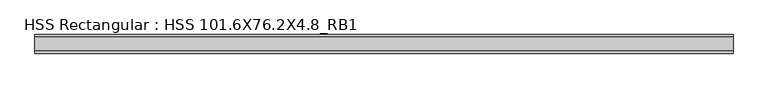
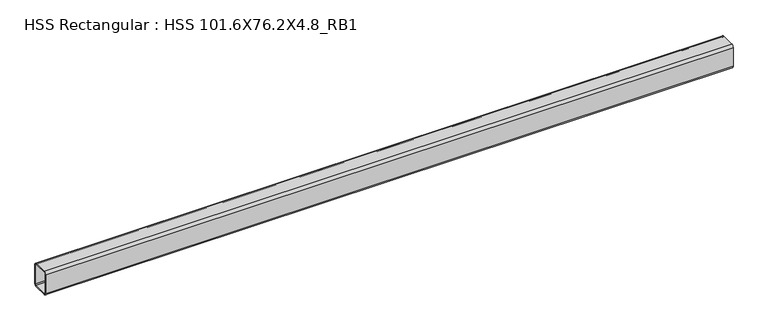
"""IFC4 building model written with IfcOpenShell, lengths in millimetres: beam geometry, HSS Rectangular : HSS 101.6X76.2X4.8_RB1."""

from ifc_helpers import new_model, si_unit, point, frame, frame_2d, origin, place, context, project, spatial, polyline, circle_curve, trimmed, segment, composite_curve, outline, extrude, source, transform, mapped, element, save


def hss_rectangular_hss_101_6x76_2x4_8_rb1_0483caaa(model_context):
    return source(origin(), model_context, "Body", "SweptSolid", [
        extrude(outline(composite_curve([segment(trimmed(circle_curve(frame_2d((-28.575, 41.275)), 9.525), [point((-38.1, 41.275))], [point((-28.575, 50.8))], False, "CARTESIAN"), True, "CONTINUOUS"), segment(polyline([(-28.575, 50.8), (28.575, 50.8)]), True, "CONTINUOUS"), segment(trimmed(circle_curve(frame_2d((28.575, 41.275)), 9.525), [point((28.575, 50.8))], [point((38.1, 41.275))], False, "CARTESIAN"), True, "CONTINUOUS"), segment(polyline([(38.1, 41.275), (38.1, -41.275)]), True, "CONTINUOUS"), segment(trimmed(circle_curve(frame_2d((28.575, -41.275)), 9.525), [point((38.1, -41.275))], [point((28.575, -50.8))], False, "CARTESIAN"), True, "CONTINUOUS"), segment(polyline([(28.575, -50.8), (-28.575, -50.8)]), True, "CONTINUOUS"), segment(trimmed(circle_curve(frame_2d((-28.575, -41.275)), 9.525), [point((-28.575, -50.8))], [point((-38.1, -41.275))], False, "CARTESIAN"), True, "CONTINUOUS"), segment(polyline([(-38.1, -41.275), (-38.1, 41.275)]), True, "CONTINUOUS")], self_intersect=False), holes=[composite_curve([segment(polyline([(28.575, 46.0375), (-28.575, 46.0375)]), True, "CONTINUOUS"), segment(trimmed(circle_curve(frame_2d((-28.575, 41.275)), 4.7625), [point((-28.575, 46.0375))], [point((-33.3375, 41.275))], True, "CARTESIAN"), True, "CONTINUOUS"), segment(polyline([(-33.3375, 41.275), (-33.3375, -41.275)]), True, "CONTINUOUS"), segment(trimmed(circle_curve(frame_2d((-28.575, -41.275)), 4.7625), [point((-33.3375, -41.275))], [point((-28.575, -46.0375))], True, "CARTESIAN"), True, "CONTINUOUS"), segment(polyline([(-28.575, -46.0375), (28.575, -46.0375)]), True, "CONTINUOUS"), segment(trimmed(circle_curve(frame_2d((28.575, -41.275)), 4.7625), [point((28.575, -46.0375))], [point((33.3375, -41.275))], True, "CARTESIAN"), True, "CONTINUOUS"), segment(polyline([(33.3375, -41.275), (33.3375, 41.275)]), True, "CONTINUOUS"), segment(trimmed(circle_curve(frame_2d((28.575, 41.275)), 4.7625), [point((33.3375, 41.275))], [point((28.575, 46.0375))], True, "CARTESIAN"), True, "CONTINUOUS")], self_intersect=False)]), frame((-1442.3750006, 0.0, 0.0), z_axis=(1.0, 0.0, 0.0), x_axis=(0.0, 1.0, 0.0)), (0.0, 0.0, 1.0), 2853.0000006),
    ])


if __name__ == "__main__":
    model = new_model("IFC4")
    model_context = context("Model", 3, world=origin())
    ifc_project = project(units=[si_unit("LENGTHUNIT", "METRE", prefix="MILLI")], contexts=[model_context])
    site = spatial("IfcSite", under=ifc_project)
    building = spatial("IfcBuilding", under=site)
    placement = place(None, origin())
    hss_rectangular_hss_101_6x76_2x4_8_rb1_shape = hss_rectangular_hss_101_6x76_2x4_8_rb1_0483caaa(model_context)
    element("IfcBeam", 1, ObjectType="HSS Rectangular : HSS 101.6X76.2X4.8_RB1", at=placement, inside=building, context=model_context, shape_type="MappedRepresentation", body=[
        mapped(hss_rectangular_hss_101_6x76_2x4_8_rb1_shape, transform((0.0, 0.0, 0.0), x_axis=(1.0, 0.0, 0.0), y_axis=(0.0, 1.0, 0.0), z_axis=(0.0, 0.0, 1.0))),
    ])
    save(model, "model.ifc")

# Revit data of these elements
# Type "HSS Rectangular : HSS 101.6X76.2X4.8_RB1"
#   Section Name Key = "HSS 4X3X3/16"
#   Assembly Code = "B10"
#   Width = 7.62 cm
#   Wall Nominal Thickness = 0.4763 cm
#   Wall Design Thickness = 0.442 cm
#   Torsional Moment of Inertia = 260.561 cm⁴
#   Torsional Modulus = 61.2876 cm³
#   Section Area = 14.4516 cm²
#   Plastic Modulus weak axis = 40.3122 cm³
#   Plastic Modulus strong axis = 49.1612 cm³
#   Perimeter = 0.881482 m²/m
#   Outer Fillet = 0.9525 cm
#   Nominal Weight = 12.1285 kgf/m
#   Moment of Inertia weak axis = 131.529 cm⁴
#   Moment of Inertia strong axis = 205.202 cm⁴
#   Inner Fillet = 0.4763 cm
#   Height = 10.16 cm
#   Elastic Modulus weak axis = 34.4128 cm³
#   Elastic Modulus strong axis = 40.476 cm³
#   Centroid Vertical = 5.08 cm
#   Centroid Horizontal = 3.81 cm
#   Length [instance default] = 1524 mm
#   Structural Material [instance default] = Steel ASTM A500, Grade B, Rectangular and Square
#   Principal Axes Angle = 0
# Element 1 (IfcBeam, "HSS Rectangular : HSS 101.6X76.2X4.8_RB1")
#   Structural Material = Steel ASTM A992
#   Materials on its faces: "Steel ASTM A992"
# Materials
#   "Steel ASTM A500, Grade B, Rectangular and Square": class "Metal", colour RGB 199 199 199, transparency 0, Description = "Carbon steel", Cost = 0
#   "Steel ASTM A992": class "Metal", colour RGB 199 199 199, transparency 0, Description = "Structural steel 50ksi", Cost = 0
